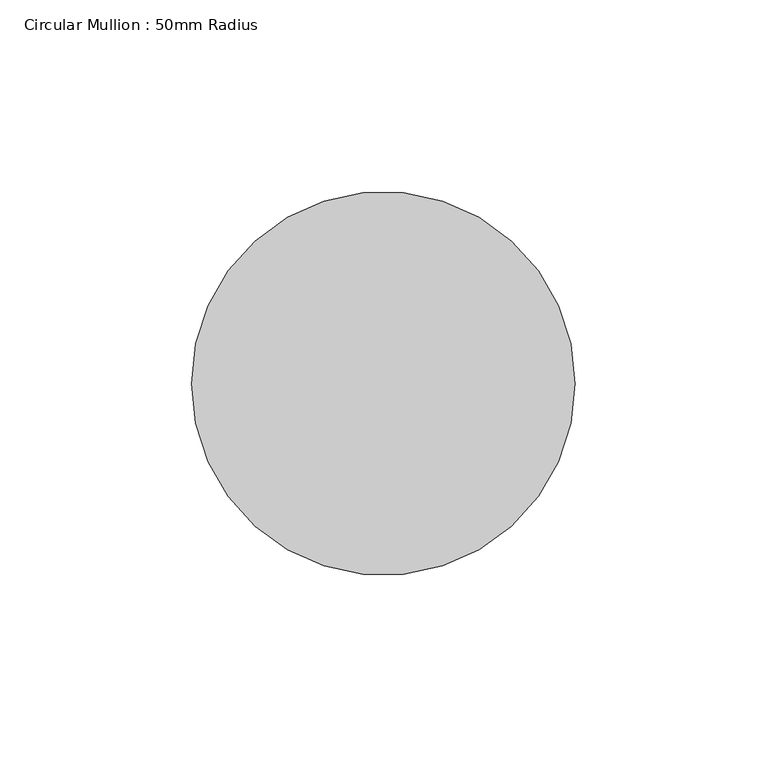
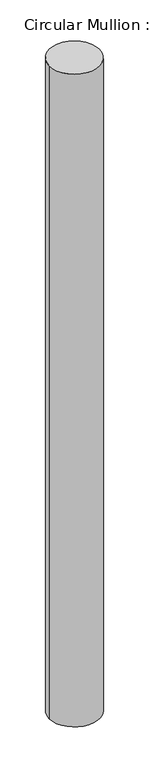
"""IFC4 building model written with IfcOpenShell, lengths in millimetres: member geometry, Circular Mullion : 50mm Radius."""

from ifc_helpers import new_model, si_unit, point, frame, origin, origin_2d, place, context, project, spatial, circle_curve, trimmed, segment, composite_curve, outline, extrude, source, transform, mapped, element, save


def circular_mullion_50mm_radius_17f5e407(model_context):
    return source(origin(), model_context, "Body", "SweptSolid", [
        extrude(outline(composite_curve([segment(trimmed(circle_curve(origin_2d(), 50.0), [point((50.0, 0.0))], [point((-50.0, 0.0))], False, "CARTESIAN"), True, "CONTINUOUS"), segment(trimmed(circle_curve(origin_2d(), 50.0), [point((-50.0, 0.0))], [point((50.0, 0.0))], False, "CARTESIAN"), True, "CONTINUOUS")], self_intersect=False)), frame((0.0, 0.0, -1372.7521036), z_axis=(0.0, 0.0, 1.0), x_axis=(1.0, 0.0, 0.0)), (0.0, 0.0, 1.0), 1372.7521036),
    ])


if __name__ == "__main__":
    model = new_model("IFC4")
    model_context = context("Model", 3, world=origin())
    ifc_project = project(units=[si_unit("LENGTHUNIT", "METRE", prefix="MILLI")], contexts=[model_context])
    site = spatial("IfcSite", under=ifc_project)
    building = spatial("IfcBuilding", under=site)
    placement = place(None, origin())
    circular_mullion_50mm_radius_shape = circular_mullion_50mm_radius_17f5e407(model_context)
    element("IfcMember", 1, ObjectType="Circular Mullion : 50mm Radius", at=placement, inside=building, context=model_context, shape_type="MappedRepresentation", body=[
        mapped(circular_mullion_50mm_radius_shape, transform((0.0, 0.0, 0.0), x_axis=(1.0, 0.0, 0.0), y_axis=(0.0, 1.0, 0.0), z_axis=(0.0, 0.0, 1.0))),
    ])
    save(model, "model.ifc")

# Revit data of these elements
# Type "Circular Mullion : 50mm Radius"
#   built-in parameter 1007350 = 0.164042 (stored number, unit not read)
# Element 1 (IfcMember, "Circular Mullion : 50mm Radius")
#   Materials on its faces: "Aluminium"
# Materials
#   "Aluminium": class "Metal", colour RGB 247 247 247, transparency 0, Description = "Aluminium 6061", Cost = 0
